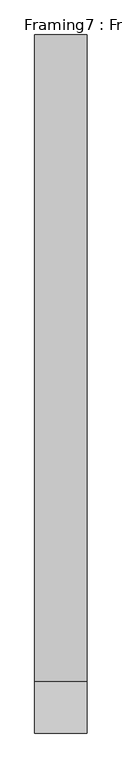
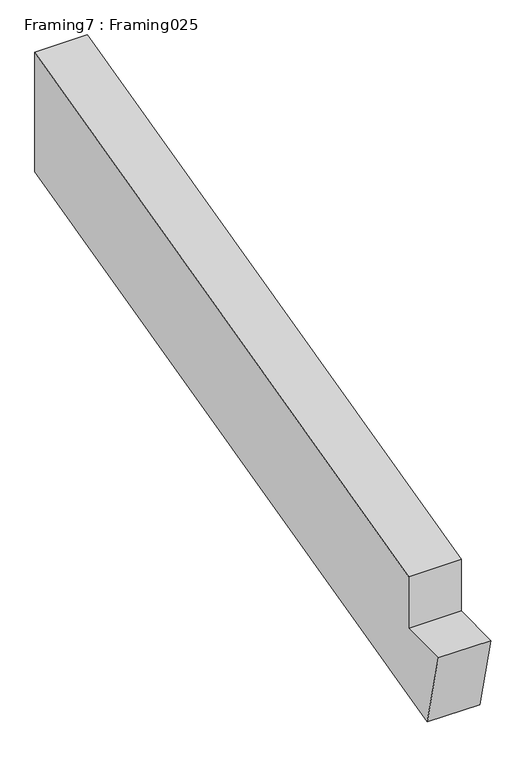
"""IFC4 building model written with IfcOpenShell, lengths in millimetres: proxy geometry, Framing7 : Framing025."""

from ifc_helpers import new_model, si_unit, frame, origin, place, context, project, spatial, polyline, outline, extrude, source, transform, mapped, element, save


def framing7_framing025_fdaa2fb1(model_context):
    return source(origin(), model_context, "Body", "SweptSolid", [
        extrude(outline(polyline([(-5374.9745897, 42642.0307603), (-5224.4076049, 42642.0307603), (-5224.4076049, 42800.8143799), (-3344.6566162, 43270.717426), (-3344.6566162, 42903.8818003), (-5318.455674, 42411.3663805), (-5374.9745897, 42642.0307603)])), frame((12534.9, 0.0, 0.0), z_axis=(1.0, 0.0, 0.0), x_axis=(0.0, 1.0, 0.0)), (0.0, 0.0, 1.0), 152.4),
    ])


if __name__ == "__main__":
    model = new_model("IFC4")
    model_context = context("Model", 3, world=origin())
    ifc_project = project(units=[si_unit("LENGTHUNIT", "METRE", prefix="MILLI")], contexts=[model_context])
    site = spatial("IfcSite", under=ifc_project)
    building = spatial("IfcBuilding", under=site)
    placement = place(None, origin())
    framing7_framing025_shape = framing7_framing025_fdaa2fb1(model_context)
    element("IfcBuildingElementProxy", 1, Name="Framing7 : Framing025", ObjectType="Framing7 : Framing025", at=placement, inside=building, context=model_context, shape_type="MappedRepresentation", body=[
        mapped(framing7_framing025_shape, transform((0.0, 0.0, 0.0), x_axis=(1.0, 0.0, 0.0), y_axis=(0.0, 1.0, 0.0), z_axis=(0.0, 0.0, 1.0))),
    ])
    save(model, "model.ifc")

# Revit data of these elements
# Type "Framing7 : Framing025"
#   NameOverride = "Framing025"
# Element 1 (IfcBuildingElementProxy, "Framing7 : Framing025")
#   Materials on its faces: "WOOD FRAMING (SEE STRUCT DWGS)"
# Materials
#   "WOOD FRAMING (SEE STRUCT DWGS)": class "Unassigned", colour RGB 224 188 168, transparency 0, Cost = 0
